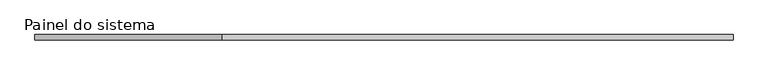
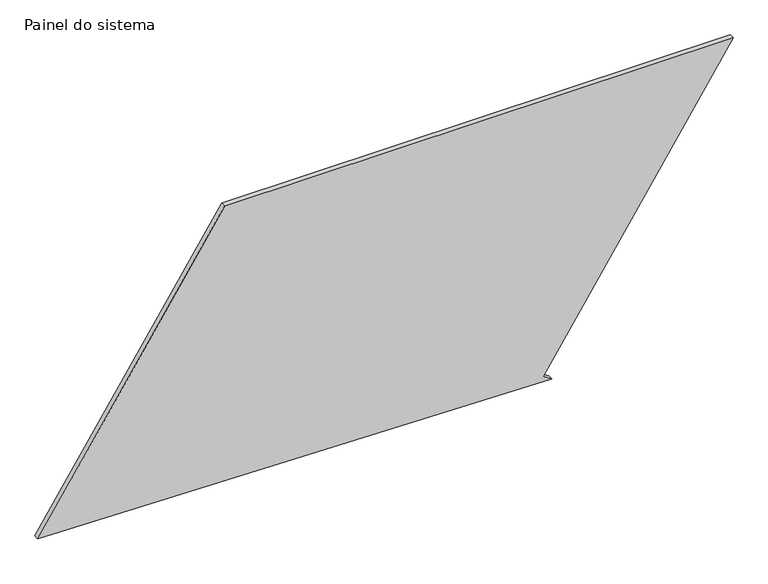
"""IFC4 building model written with IfcOpenShell, lengths in millimetres: plate geometry, Painel do sistema : Envidraçado."""

from ifc_helpers import new_model, si_unit, frame, origin, place, context, project, spatial, polyline, outline, extrude, source, transform, mapped, element, save


def painel_do_sistema_7ec283e2(model_context):
    return source(origin(), model_context, "Body", "SweptSolid", [
        extrude(outline(polyline([(0.0, 804.8329705), (27.2709308, 762.9247812), (1438.8862565, 1681.5057195), (1438.8862565, -778.4613269), (51.1464818, -1681.5057195), (0.0, 804.8329705)])), frame((0.0, 24.5, 0.0), z_axis=(0.0, 1.0, 0.0), x_axis=(0.0, 0.0, 1.0)), (0.0, 0.0, 1.0), 25.0),
    ])


if __name__ == "__main__":
    model = new_model("IFC4")
    model_context = context("Model", 3, world=origin())
    ifc_project = project(units=[si_unit("LENGTHUNIT", "METRE", prefix="MILLI")], contexts=[model_context])
    site = spatial("IfcSite", under=ifc_project)
    building = spatial("IfcBuilding", under=site)
    placement = place(None, origin())
    painel_do_sistema_shape = painel_do_sistema_7ec283e2(model_context)
    element("IfcPlate", 1, ObjectType="Painel do sistema : Envidraçado", at=placement, inside=building, context=model_context, shape_type="MappedRepresentation", body=[
        mapped(painel_do_sistema_shape, transform((0.0, 0.0, 0.0), x_axis=(1.0, 0.0, 0.0), y_axis=(0.0, 1.0, 0.0), z_axis=(0.0, 0.0, 1.0))),
    ])
    save(model, "model.ifc")

# Revit data of these elements
# Type "Painel do sistema : Envidraçado"
#   Construction Type Id = "GSP4R"
#   Analytic Construction = "Vidraça única Pilkington 1/8 pol"
#   Visual Light Transmittance = 0.9
#   Solar Heat Gain Coefficient = 0.86
#   Heat Transfer Coefficient (U) = 6.7069 W/(m²·K)
# Element 1 (IfcPlate, "Painel do sistema : Envidraçado")
#   Materials on its faces: "Vidro"
# Materials
#   "Vidro": class "Vidro", colour RGB 0 128 192, transparency 0.9, Description = "Vidro de sílica", Cost = 0
